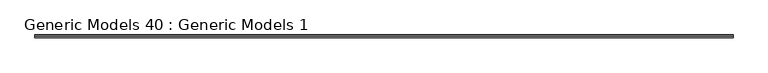
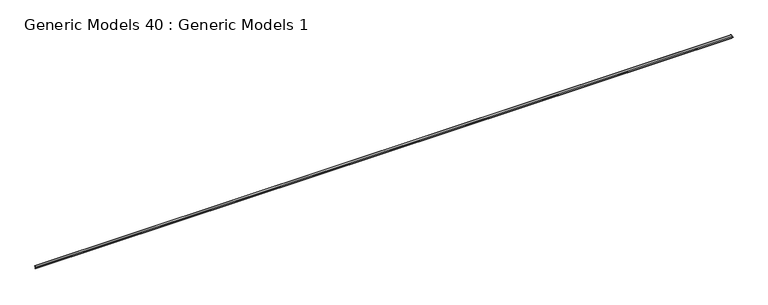
"""IFC4 building model written with IfcOpenShell, lengths in millimetres: proxy geometry, Generic Models 40 : Generic Models 1."""

import ifcopenshell
import ifcopenshell.guid

model = None  # the IFC model being written
_history = None  # IfcOwnerHistory: only IFC2X3 demands one
_inside = {}  # id of a spatial element -> (the spatial element, [elements in it])
_under = {}  # id of a project, library or spatial element -> (it, [spatial elements below it])
_declared = {}  # id of a project -> (the project, [libraries it declares])
_typed = {}  # id of a type object -> (the type object, [elements of that type])
_made_of = {}  # id of a material, layer set ... -> (it, [elements and type objects made of it])


def new_model(schema):
    """Start an empty IFC model of exactly this schema.

    Asked for "IFC4X3", IfcOpenShell would pick the latest addendum, in which some entities
    have other attributes; the version numbers below select the first issue.
    IFC2X3 requires an IfcOwnerHistory on every rooted entity: one is made here for all.
    """
    global model, _history
    if schema == "IFC4X3":
        model = ifcopenshell.file(schema_version=(4, 3, 0, 0))
    else:
        model = ifcopenshell.file(schema=schema)
    _inside.clear()
    _under.clear()
    _declared.clear()
    _typed.clear()
    _made_of.clear()
    _history = None
    if model.schema == "IFC2X3":
        org = make("IfcOrganization", Name="unknown")
        user = make(
            "IfcPersonAndOrganization",
            ThePerson=make("IfcPerson", FamilyName="unknown"),
            TheOrganization=org,
        )
        app = make(
            "IfcApplication",
            ApplicationDeveloper=org,
            Version="unknown",
            ApplicationFullName="unknown",
            ApplicationIdentifier="unknown",
        )
        _history = make(
            "IfcOwnerHistory",
            OwningUser=user,
            OwningApplication=app,
            ChangeAction="ADDED",
            CreationDate=0,
        )
    return model


def make(cls, **values):
    """One entity of the class cls with the attributes given. An attribute that is None is left unset."""
    return model.create_entity(
        cls, **{name: value for name, value in values.items() if value is not None}
    )


def rooted(cls, **values):
    """An entity with a GlobalId (a new one), such as an element, a storey or a relation."""
    return make(cls, GlobalId=ifcopenshell.guid.new(), OwnerHistory=_history, **values)


def si_unit(unit_type, name, prefix=None):
    """IfcSIUnit, for example si_unit("LENGTHUNIT", "METRE", prefix="MILLI")."""
    return make("IfcSIUnit", UnitType=unit_type, Prefix=prefix, Name=name)


def assignment(units):
    """IfcUnitAssignment: the units of a project."""
    return None if units is None else make("IfcUnitAssignment", Units=units)


def point(xyz):
    """IfcCartesianPoint."""
    return None if xyz is None else make("IfcCartesianPoint", Coordinates=xyz)


def direction(xyz):
    """IfcDirection."""
    return None if xyz is None else make("IfcDirection", DirectionRatios=xyz)


def frame(location, z_axis=None, x_axis=None):
    """IfcAxis2Placement3D, a coordinate frame: its origin and axes. An axis left out is left unset."""
    return make(
        "IfcAxis2Placement3D",
        Location=point(location),
        Axis=direction(z_axis),
        RefDirection=direction(x_axis),
    )


def frame_2d(location, x_axis=None):
    """IfcAxis2Placement2D, a coordinate frame in the plane: its origin and x axis."""
    return make(
        "IfcAxis2Placement2D", Location=point(location), RefDirection=direction(x_axis)
    )


def origin():
    """The frame at (0, 0, 0) with its axes left unset."""
    return frame((0.0, 0.0, 0.0))


def place(relative_to, where):
    """IfcLocalPlacement: puts the frame where relative to a parent placement (None: the world)."""
    return make(
        "IfcLocalPlacement", PlacementRelTo=relative_to, RelativePlacement=where
    )


def context(
    kind, dimensions, precision=None, world=None, true_north=None, identifier=None
):
    """IfcGeometricRepresentationContext, for example the 3D "Model" context."""
    return make(
        "IfcGeometricRepresentationContext",
        ContextIdentifier=identifier,
        ContextType=kind,
        CoordinateSpaceDimension=dimensions,
        Precision=precision,
        WorldCoordinateSystem=world,
        TrueNorth=true_north,
    )


def project(units=None, contexts=None):
    """IfcProject with its units and contexts."""
    return rooted(
        "IfcProject",
        Name="project",
        RepresentationContexts=contexts,
        UnitsInContext=assignment(units),
    )


def spatial(cls, under=None, at=None, **own):
    """A site, building, storey or space (cls), placed at a placement, below another one or the project."""
    s = rooted(cls, ObjectPlacement=at, **own)
    if under is not None:
        _under.setdefault(under.id(), (under, []))[1].append(s)
    return s


def polyline(points):
    """IfcPolyline through the points."""
    return make("IfcPolyline", Points=[point(p) for p in points])


def circle_curve(where, radius):
    """IfcCircle in the frame where."""
    return make("IfcCircle", Position=where, Radius=radius)


def trimmed(basis, trim1, trim2, sense, master):
    """IfcTrimmedCurve: the piece of a basis curve between two trims."""
    return make(
        "IfcTrimmedCurve",
        BasisCurve=basis,
        Trim1=trim1,
        Trim2=trim2,
        SenseAgreement=sense,
        MasterRepresentation=master,
    )


def segment(curve, same_sense, transition):
    """IfcCompositeCurveSegment."""
    return make(
        "IfcCompositeCurveSegment",
        Transition=transition,
        SameSense=same_sense,
        ParentCurve=curve,
    )


def composite_curve(segments, self_intersect=None):
    """IfcCompositeCurve: segments joined end to end."""
    return make("IfcCompositeCurve", Segments=segments, SelfIntersect=self_intersect)


def outline(outer, holes=None, kind="AREA"):
    """IfcArbitraryClosedProfileDef: a profile drawn as a closed curve; with holes, ...WithVoids."""
    if holes is None:
        return make("IfcArbitraryClosedProfileDef", ProfileType=kind, OuterCurve=outer)
    return make(
        "IfcArbitraryProfileDefWithVoids",
        ProfileType=kind,
        OuterCurve=outer,
        InnerCurves=holes,
    )


def extrude(swept, where, along, depth):
    """IfcExtrudedAreaSolid: the profile swept, set in the frame where, extruded along a direction by depth."""
    return make(
        "IfcExtrudedAreaSolid",
        SweptArea=swept,
        Position=where,
        ExtrudedDirection=direction(along),
        Depth=depth,
    )


def shape(context_of_items, identifier, shape_type, items):
    """IfcShapeRepresentation: the items that make up one representation, for example the "Body"."""
    return make(
        "IfcShapeRepresentation",
        ContextOfItems=context_of_items,
        RepresentationIdentifier=identifier,
        RepresentationType=shape_type,
        Items=items,
    )


def source(mapping_origin, context_of_items, identifier, shape_type, items):
    """IfcRepresentationMap: a shape defined once, which mapped items show again and again."""
    return make(
        "IfcRepresentationMap",
        MappingOrigin=mapping_origin,
        MappedRepresentation=shape(context_of_items, identifier, shape_type, items),
    )


def transform(
    local_origin,
    x_axis=None,
    y_axis=None,
    z_axis=None,
    scale=None,
    scale2=None,
    scale3=None,
    uniform=True,
):
    """IfcCartesianTransformationOperator3D, or its non-uniform kind. x_axis, y_axis, z_axis: its Axis1, 2, 3."""
    if uniform:
        return make(
            "IfcCartesianTransformationOperator3D",
            Axis1=direction(x_axis),
            Axis2=direction(y_axis),
            LocalOrigin=point(local_origin),
            Scale=scale,
            Axis3=direction(z_axis),
        )
    return make(
        "IfcCartesianTransformationOperator3DnonUniform",
        Axis1=direction(x_axis),
        Axis2=direction(y_axis),
        LocalOrigin=point(local_origin),
        Scale=scale,
        Axis3=direction(z_axis),
        Scale2=scale2,
        Scale3=scale3,
    )


def mapped(mapping_source, mapping_target):
    """IfcMappedItem: shows the shape of a source again, moved by a transform."""
    return make(
        "IfcMappedItem", MappingSource=mapping_source, MappingTarget=mapping_target
    )


def made_of(thing, what):
    """Note that an element or type object is made of a material, layer set ...; save() writes the relation."""
    if what is not None:
        _made_of.setdefault(what.id(), (what, []))[1].append(thing)
    return thing


def element(
    cls,
    number,
    at=None,
    inside=None,
    cuts=None,
    type_object=None,
    material=None,
    context=None,
    identifier="Body",
    shape_type=None,
    held_by="IfcProductDefinitionShape",
    body=None,
    shapes=None,
    **own,
):
    """One element of the class cls, such as IfcWall. Its Tag is "e" and its number.

    at: its placement. inside: the storey or other place that contains it. cuts: it is an
    opening in that element (IfcRelVoidsElement). A single representation is given by context,
    identifier, shape_type and body (its items); several are given by shapes. held_by: the class
    of the entity that holds the representations. save() writes the other relations.
    """
    e = rooted(cls, Tag="e%d" % number, ObjectPlacement=at, **own)
    if body is not None:
        shapes = [shape(context, identifier, shape_type, body)]
    if shapes is not None:
        e.Representation = make(held_by, Representations=shapes)
    if inside is not None:
        _inside.setdefault(inside.id(), (inside, []))[1].append(e)
    if cuts is not None:
        rooted(
            "IfcRelVoidsElement", RelatingBuildingElement=cuts, RelatedOpeningElement=e
        )
    if type_object is not None:
        _typed.setdefault(type_object.id(), (type_object, []))[1].append(e)
    return made_of(e, material)


def aggregate(whole, parts):
    """IfcRelAggregates: a whole, such as a stair, and the parts it consists of."""
    return rooted("IfcRelAggregates", RelatingObject=whole, RelatedObjects=parts)


def save(model, path):
    """Write the relations noted so far, then the file.

    IfcRelAggregates (storeys below a building ...), IfcRelContainedInSpatialStructure (elements
    in a storey), IfcRelDefinesByType, IfcRelAssociatesMaterial and IfcRelDeclares: one each for
    every whole, place, type object, material and project.
    """
    for whole, parts in _under.values():
        aggregate(whole, parts)
    for where, things in _inside.values():
        rooted(
            "IfcRelContainedInSpatialStructure",
            RelatedElements=things,
            RelatingStructure=where,
        )
    for kind, things in _typed.values():
        rooted("IfcRelDefinesByType", RelatedObjects=things, RelatingType=kind)
    for what, things in _made_of.values():
        rooted("IfcRelAssociatesMaterial", RelatedObjects=things, RelatingMaterial=what)
    for by, libraries in _declared.values():
        rooted("IfcRelDeclares", RelatingContext=by, RelatedDefinitions=libraries)
    model.write(path)


def generic_models_40_generic_models_1_98de381b(model_context):
    return source(origin(), model_context, "Body", "SweptSolid", [
        extrude(outline(composite_curve([segment(trimmed(circle_curve(frame_2d((14317.8032532, 127165.3167873)), 1.4342127), [point((14317.1480982, 127166.5926156))], [point((14319.0790815, 127164.6616323))], False, "CARTESIAN"), True, "CONTINUOUS"), segment(polyline([(14319.0790815, 127164.6616323), (14299.5524659, 127126.6361176), (14299.5524659, 127088.5361176), (14298.2824659, 127088.5361176), (14298.2824659, 127126.9431414), (14318.1827056, 127165.6962396), (14279.4296073, 127145.796), (14241.0225835, 127145.796), (14241.0225835, 127147.066), (14279.1225835, 127147.066), (14317.1480982, 127166.5926156)]), True, "CONTINUOUS")], self_intersect=False)), frame((-20998.9733045, 0.0, 0.0), z_axis=(1.0, 0.0, 0.0), x_axis=(0.0, 1.0, 0.0)), (0.0, 0.0, 1.0), 19050.0),
    ])


if __name__ == "__main__":
    model = new_model("IFC4")
    model_context = context("Model", 3, world=origin())
    ifc_project = project(units=[si_unit("LENGTHUNIT", "METRE", prefix="MILLI")], contexts=[model_context])
    site = spatial("IfcSite", under=ifc_project)
    building = spatial("IfcBuilding", under=site)
    placement = place(None, origin())
    generic_models_40_generic_models_1_shape = generic_models_40_generic_models_1_98de381b(model_context)
    element("IfcBuildingElementProxy", 1, Name="Generic Models 40 : Generic Models 1", ObjectType="Generic Models 40 : Generic Models 1", at=placement, inside=building, context=model_context, shape_type="MappedRepresentation", body=[
        mapped(generic_models_40_generic_models_1_shape, transform((0.0, 0.0, 0.0), x_axis=(1.0, 0.0, 0.0), y_axis=(0.0, 1.0, 0.0), z_axis=(0.0, 0.0, 1.0))),
    ])
    save(model, "model.ifc")

# Revit data of these elements
# Element 1 (IfcBuildingElementProxy, "Generic Models 40 : Generic Models 1")
#   Materials on its faces: "_CONTINIOUS 16 GA. COPPER CORNER BEAD"
# Materials
#   "_CONTINIOUS 16 GA. COPPER CORNER BEAD": class "Generic", colour RGB 253 192 103, transparency 0, Cost = 0
